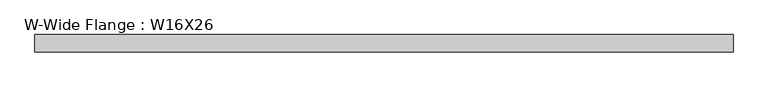
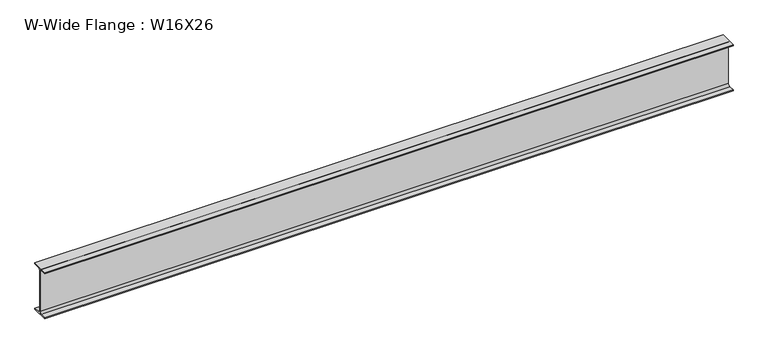
"""IFC4 building model written with IfcOpenShell, lengths in millimetres: beam geometry, W-Wide Flange : W16X26."""

from ifc_helpers import new_model, si_unit, point, frame, frame_2d, origin, place, context, project, spatial, polyline, circle_curve, trimmed, segment, composite_curve, outline, extrude, source, transform, mapped, element, save


def w_wide_flange_w16x26_169e22ba(model_context):
    return source(origin(), model_context, "Body", "SweptSolid", [
        extrude(outline(composite_curve([segment(polyline([(69.85, -190.627), (69.85, -199.39), (-69.85, -199.39), (-69.85, -190.627), (-21.3995, -190.627)]), True, "CONTINUOUS"), segment(trimmed(circle_curve(frame_2d((-21.3995, -172.4025)), 18.2245), [point((-21.3995, -190.627))], [point((-3.175, -172.4025))], True, "CARTESIAN"), True, "CONTINUOUS"), segment(polyline([(-3.175, -172.4025), (-3.175, 172.4025)]), True, "CONTINUOUS"), segment(trimmed(circle_curve(frame_2d((-21.3995, 172.4025)), 18.2245), [point((-3.175, 172.4025))], [point((-21.3995, 190.627))], True, "CARTESIAN"), True, "CONTINUOUS"), segment(polyline([(-21.3995, 190.627), (-69.85, 190.627), (-69.85, 199.39), (69.85, 199.39), (69.85, 190.627), (21.3995, 190.627)]), True, "CONTINUOUS"), segment(trimmed(circle_curve(frame_2d((21.3995, 172.4025)), 18.2245), [point((21.3995, 190.627))], [point((3.175, 172.4025))], True, "CARTESIAN"), True, "CONTINUOUS"), segment(polyline([(3.175, 172.4025), (3.175, -172.4025)]), True, "CONTINUOUS"), segment(trimmed(circle_curve(frame_2d((21.3995, -172.4025)), 18.2245), [point((3.175, -172.4025))], [point((21.3995, -190.627))], True, "CARTESIAN"), True, "CONTINUOUS"), segment(polyline([(21.3995, -190.627), (69.85, -190.627)]), True, "CONTINUOUS")], self_intersect=False)), frame((-2806.7, 0.0, 0.0), z_axis=(1.0, 0.0, 0.0), x_axis=(0.0, 1.0, 0.0)), (0.0, 0.0, 1.0), 5613.4),
    ])


if __name__ == "__main__":
    model = new_model("IFC4")
    model_context = context("Model", 3, world=origin())
    ifc_project = project(units=[si_unit("LENGTHUNIT", "METRE", prefix="MILLI")], contexts=[model_context])
    site = spatial("IfcSite", under=ifc_project)
    building = spatial("IfcBuilding", under=site)
    placement = place(None, origin())
    w_wide_flange_w16x26_shape = w_wide_flange_w16x26_169e22ba(model_context)
    element("IfcBeam", 1, ObjectType="W-Wide Flange : W16X26", at=placement, inside=building, context=model_context, shape_type="MappedRepresentation", body=[
        mapped(w_wide_flange_w16x26_shape, transform((0.0, 0.0, 0.0), x_axis=(1.0, 0.0, 0.0), y_axis=(0.0, 1.0, 0.0), z_axis=(0.0, 0.0, 1.0))),
    ])
    save(model, "model.ifc")

# Revit data of these elements
# Type "W-Wide Flange : W16X26"
#   Assembly Code = "B10"
#   W = 26
#   Length [instance default] = 5' - 0"
#   bf = 0' - 5 1/2"
#   d = 1' - 3.7"
#   k = 0' - 1 1/16"
#   k2 = 0' - 0.7175"
#   tf = 0' - 0.345"
#   tw = 0' - 0 1/4"
#   A = 0.0533333 SF
#   Structural Material [instance default] = Steel ASTM A992
# Element 1 (IfcBeam, "W-Wide Flange : W16X26")
#   Materials on its faces: "Steel ASTM A992"
# Materials
#   "Steel ASTM A992": class "Metal", colour RGB 199 199 199, transparency 0, Description = "Structural steel 50ksi", Cost = 0
